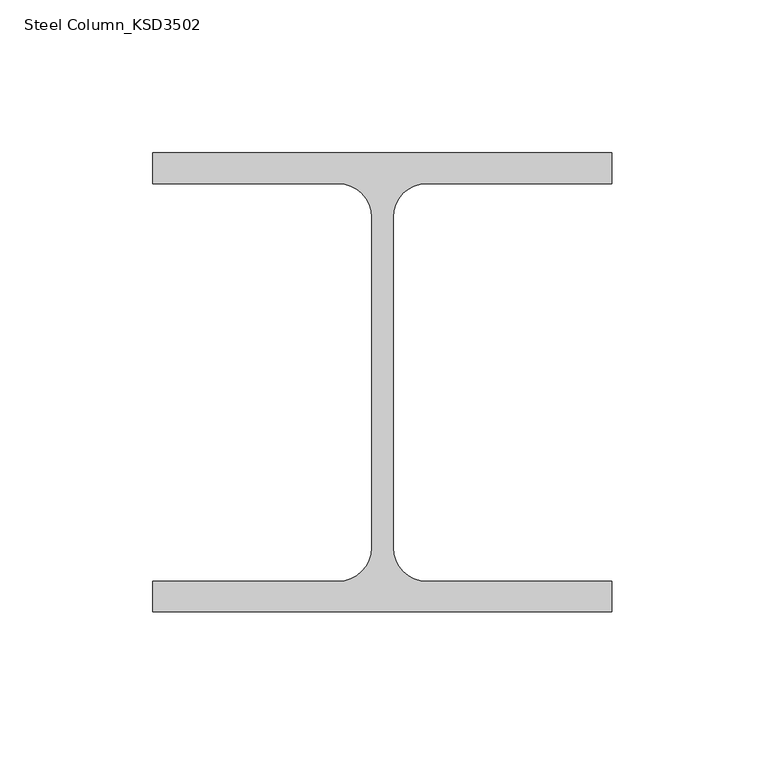
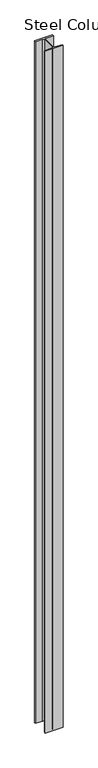
"""IFC4 building model written with IfcOpenShell, lengths in millimetres: column geometry, Steel Column_KSD3502 : H_SC_ASC_H-150×150x7x10."""

from ifc_helpers import new_model, si_unit, point, frame, frame_2d, origin, place, context, project, spatial, polyline, circle_curve, trimmed, segment, composite_curve, outline, extrude, source, transform, mapped, element, save


def steel_column_ksd3502_5fc823e1(model_context):
    return source(origin(), model_context, "Body", "SweptSolid", [
        extrude(outline(composite_curve([segment(polyline([(75.0, 75.0), (75.0, 65.0), (14.5, 65.0)]), True, "CONTINUOUS"), segment(trimmed(circle_curve(frame_2d((14.5, 54.0)), 11.0), [point((14.5, 65.0))], [point((3.5, 54.0))], True, "CARTESIAN"), True, "CONTINUOUS"), segment(polyline([(3.5, 54.0), (3.5, -54.0)]), True, "CONTINUOUS"), segment(trimmed(circle_curve(frame_2d((14.5, -54.0)), 11.0), [point((3.5, -54.0))], [point((14.5, -65.0))], True, "CARTESIAN"), True, "CONTINUOUS"), segment(polyline([(14.5, -65.0), (75.0, -65.0), (75.0, -75.0), (-75.0, -75.0), (-75.0, -65.0), (-14.5, -65.0)]), True, "CONTINUOUS"), segment(trimmed(circle_curve(frame_2d((-14.5, -54.0)), 11.0), [point((-14.5, -65.0))], [point((-3.5, -54.0))], True, "CARTESIAN"), True, "CONTINUOUS"), segment(polyline([(-3.5, -54.0), (-3.5, 54.0)]), True, "CONTINUOUS"), segment(trimmed(circle_curve(frame_2d((-14.5, 54.0)), 11.0), [point((-3.5, 54.0))], [point((-14.5, 65.0))], True, "CARTESIAN"), True, "CONTINUOUS"), segment(polyline([(-14.5, 65.0), (-75.0, 65.0), (-75.0, 75.0), (75.0, 75.0)]), True, "CONTINUOUS")], self_intersect=False)), frame((0.0, 0.0, 599.9720055), z_axis=(0.0, 0.0, 1.0), x_axis=(1.0, 0.0, 0.0)), (0.0, 0.0, 1.0), 6000.0),
    ])


if __name__ == "__main__":
    model = new_model("IFC4")
    model_context = context("Model", 3, world=origin())
    ifc_project = project(units=[si_unit("LENGTHUNIT", "METRE", prefix="MILLI")], contexts=[model_context])
    site = spatial("IfcSite", under=ifc_project)
    building = spatial("IfcBuilding", under=site)
    placement = place(None, origin())
    steel_column_ksd3502_shape = steel_column_ksd3502_5fc823e1(model_context)
    element("IfcColumn", 1, ObjectType="Steel Column_KSD3502 : H_SC_ASC_H-150×150x7x10", at=placement, inside=building, context=model_context, shape_type="MappedRepresentation", body=[
        mapped(steel_column_ksd3502_shape, transform((0.0, 0.0, 0.0), x_axis=(1.0, 0.0, 0.0), y_axis=(0.0, 1.0, 0.0), z_axis=(0.0, 0.0, 1.0))),
    ])
    save(model, "model.ifc")

# Revit data of these elements
# Type "Steel Column_KSD3502 : H_SC_ASC_H-150×150x7x10"
#   Width = 15.0 cm
#   Web Thickness = 0.7 cm
#   Web Fillet = 1.1 cm
#   Warping Constant = 27562.5 cm⁶
#   Torsional Moment of Inertia = 11.6007 cm⁴
#   Section Area = 40.14 cm²
#   Plastic Modulus weak axis = 115.0 cm³
#   Plastic Modulus strong axis = 246.0 cm³
#   Perimeter = 1.27 m²/m
#   Nominal Weight = 31.50 kgf/m
#   Moment of Inertia weak axis = 563.00 cm⁴
#   Moment of Inertia strong axis = 1640.00 cm⁴
#   Height = 15.0 cm
#   Flange Thickness = 1.0 cm
#   Elastic Modulus weak axis = 75.1 cm³
#   Elastic Modulus strong axis = 219.0 cm³
#   Centroid Vertical = 7.5 cm
#   Centroid Horizontal = 7.5 cm
#   Bolt Spacing = 13.97 cm
#   Structural Material [instance default] = Steel, 45-345
#   Section Name Key = ""
#   Assembly Code = ""
# Element 1 (IfcColumn, "Steel Column_KSD3502 : H_SC_ASC_H-150×150x7x10")
#   Structural Material = A03AD029-00005_Anchor Bolt (Installation only)_M24
#   Materials on its faces: "A03AD029-00005_Anchor Bolt (Installation only)_M24"
# Materials
#   "Steel, 45-345": class "Metal", colour RGB 189 187 185, transparency 0, Description = "Steel 345 MPa", Cost = 0
#   "A03AD029-00005_Anchor Bolt (Installation only)_M24": class "Unassigned", colour RGB 84 83 81, transparency 0, Cost = 0
